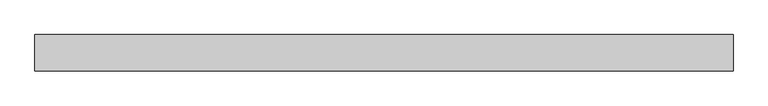
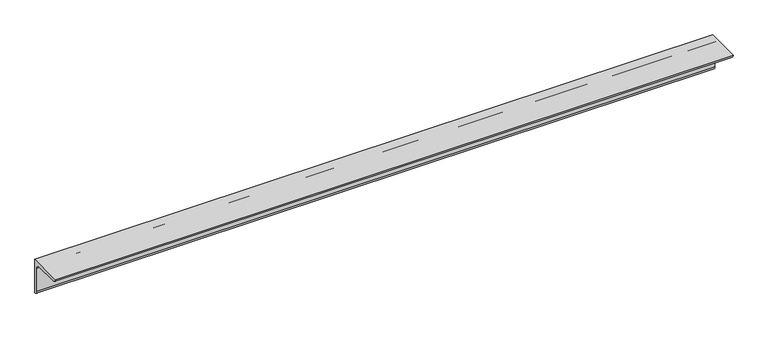
"""IFC4 building model written with IfcOpenShell, lengths in millimetres: beam geometry, 0912_Steel Framing_L-KSD3502 : H_SB_AR_S04_L-100x100x10_KBR2."""

from ifc_helpers import new_model, si_unit, point, frame, frame_2d, origin, place, context, project, spatial, polyline, circle_curve, trimmed, segment, composite_curve, outline, extrude, source, transform, mapped, element, save


def beam_98705e42(model_context):
    return source(origin(), model_context, "Body", "SweptSolid", [
        extrude(outline(composite_curve([segment(polyline([(28.2, 28.2), (28.2, -71.8)]), True, "CONTINUOUS"), segment(trimmed(circle_curve(frame_2d((28.2, -61.8)), 10.0), [point((28.2, -71.8))], [point((18.2, -61.8))], False, "CARTESIAN"), True, "CONTINUOUS"), segment(polyline([(18.2, -61.8), (18.2, 8.2)]), True, "CONTINUOUS"), segment(trimmed(circle_curve(frame_2d((8.2, 8.2)), 10.0), [point((18.2, 8.2))], [point((8.2, 18.2))], True, "CARTESIAN"), True, "CONTINUOUS"), segment(polyline([(8.2, 18.2), (-61.8, 18.2)]), True, "CONTINUOUS"), segment(trimmed(circle_curve(frame_2d((-61.8, 28.2)), 10.0), [point((-61.8, 18.2))], [point((-71.8, 28.2))], False, "CARTESIAN"), True, "CONTINUOUS"), segment(polyline([(-71.8, 28.2), (28.2, 28.2)]), True, "CONTINUOUS")], self_intersect=False)), frame((-925.8352801, 0.0, 0.0), z_axis=(1.0, 0.0, 0.0), x_axis=(0.0, 1.0, 0.0)), (0.0, 0.0, 1.0), 1920.9670248),
    ])


if __name__ == "__main__":
    model = new_model("IFC4")
    model_context = context("Model", 3, world=origin())
    ifc_project = project(units=[si_unit("LENGTHUNIT", "METRE", prefix="MILLI")], contexts=[model_context])
    site = spatial("IfcSite", under=ifc_project)
    building = spatial("IfcBuilding", under=site)
    placement = place(None, origin())
    beam_shape = beam_98705e42(model_context)
    element("IfcBeam", 1, ObjectType="0912_Steel Framing_L-KSD3502 : H_SB_AR_S04_L-100x100x10_KBR2", at=placement, inside=building, context=model_context, shape_type="MappedRepresentation", body=[
        mapped(beam_shape, transform((0.0, 0.0, 0.0), x_axis=(1.0, 0.0, 0.0), y_axis=(0.0, 1.0, 0.0), z_axis=(0.0, 0.0, 1.0))),
    ])
    save(model, "model.ifc")

# Revit data of these elements
# Type "0912_Steel Framing_L-KSD3502 : H_SB_AR_S04_L-100x100x10_KBR2"
#   k = 25 mm
#   Perimeter = 0.40 m²/m
#   Nominal Weight = 14.90 kgf/m
#   Length [instance default] = 1000 mm
#   b = 100 mm
#   d = 100 mm
#   t = 10 mm
#   x = 28.2 mm
#   y = 28.2 mm
#   A = 1900.00 m²
#   Structural Material [instance default] = Steel, 45-345
# Element 1 (IfcBeam, "0912_Steel Framing_L-KSD3502 : H_SB_AR_S04_L-100x100x10_KBR2")
#   Structural Material = Steel ASTM A36
#   Materials on its faces: "Steel ASTM A36"
# Materials
#   "Steel, 45-345": class "Metal", colour RGB 189 187 185, transparency 0, Description = "Steel 345 MPa", Cost = 0
#   "Steel ASTM A36": class "Metal", colour RGB 199 199 199, transparency 0, Description = "Structural steel, ASTM A36 Grade B, mill finish", Cost = 0
